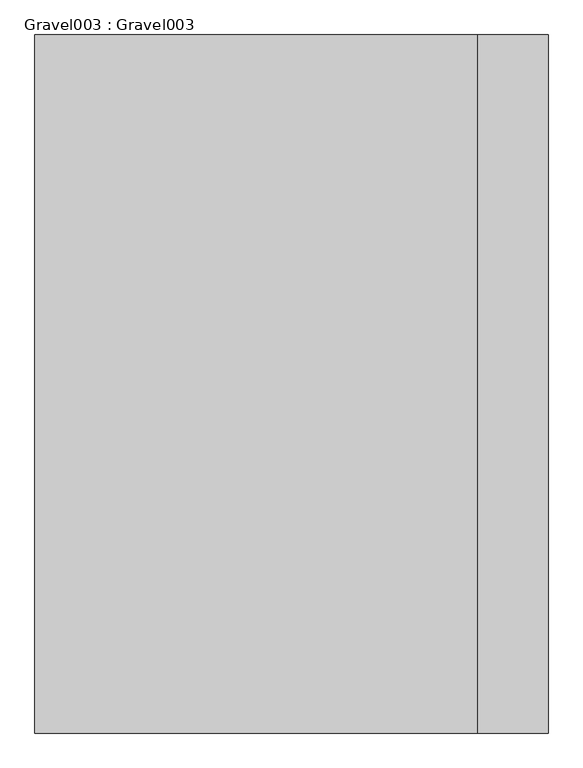
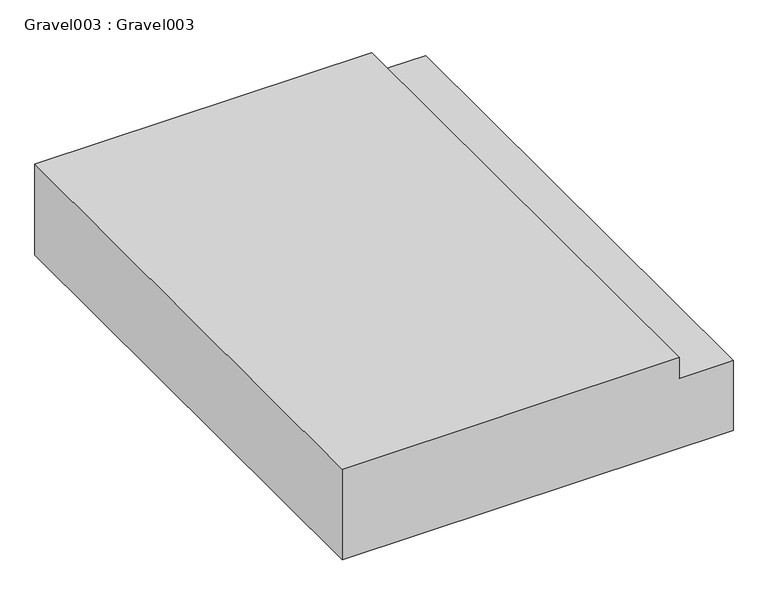
"""IFC4 building model written with IfcOpenShell, lengths in millimetres: proxy geometry, Gravel003 : Gravel003."""

from ifc_helpers import new_model, si_unit, frame, origin, place, context, project, spatial, polyline, outline, extrude, source, transform, mapped, element, save


def gravel003_gravel003_a410d6f8(model_context):
    return source(origin(), model_context, "Body", "SweptSolid", [
        extrude(outline(polyline([(32036.6025286, -10098.4737014), (32314.8961275, -10098.4737014), (32314.8961275, -10301.6737014), (32397.0602473, -10301.6737014), (32397.0602473, -11568.4300809), (32036.6025286, -11568.4300809), (32036.6025286, -10098.4737014)])), frame((0.0, 7182.1531721, 0.0), z_axis=(0.0, 1.0, 0.0), x_axis=(0.0, 0.0, 1.0)), (0.0, 0.0, 1.0), 2000.0),
    ])


if __name__ == "__main__":
    model = new_model("IFC4")
    model_context = context("Model", 3, world=origin())
    ifc_project = project(units=[si_unit("LENGTHUNIT", "METRE", prefix="MILLI")], contexts=[model_context])
    site = spatial("IfcSite", under=ifc_project)
    building = spatial("IfcBuilding", under=site)
    placement = place(None, origin())
    gravel003_gravel003_shape = gravel003_gravel003_a410d6f8(model_context)
    element("IfcBuildingElementProxy", 1, Name="Gravel003 : Gravel003", ObjectType="Gravel003 : Gravel003", at=placement, inside=building, context=model_context, shape_type="MappedRepresentation", body=[
        mapped(gravel003_gravel003_shape, transform((0.0, 0.0, 0.0), x_axis=(1.0, 0.0, 0.0), y_axis=(0.0, 1.0, 0.0), z_axis=(0.0, 0.0, 1.0))),
    ])
    save(model, "model.ifc")

# Revit data of these elements
# Type "Gravel003 : Gravel003"
#   NameOverride = "Gravel003"
# Element 1 (IfcBuildingElementProxy, "Gravel003 : Gravel003")
#   Materials on its faces: "4\" MIN. CRUSHED GRAVEL (NO FINES)"
# Materials
#   "4\" MIN. CRUSHED GRAVEL (NO FINES)": class "Unassigned", colour RGB 228 233 239, transparency 0, Cost = 0
